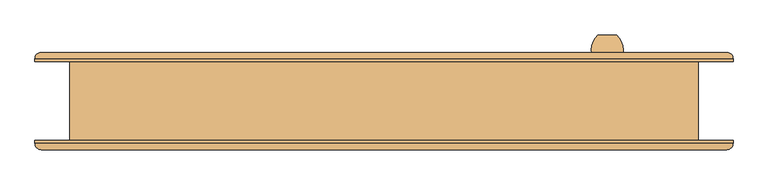
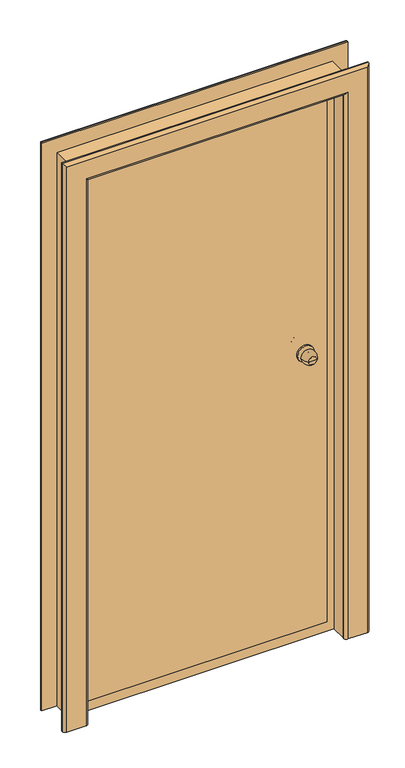
"""IFC4 building model written with IfcOpenShell, lengths in millimetres: door geometry, Наружная дверь 1-Навесная - Один проем наружу с порогом - 31173-2003 : ДСН КЛН  М1 УЗ 2100-1000 ГОСТ 31173-2003 2."""

from ifc_helpers import new_model, si_unit, point, frame, origin, place, context, project, spatial, polyline, circle_curve, ellipse_curve, trimmed, outline, extrude, faceted_brep, source, transform, mapped, element, save
from ifc_brep_helpers import plane_surface, cylinder_surface, revolved_surface, advanced_brep


def door_9195733c(model_context):
    return source(origin(), model_context, "Body", "SolidModel", [
        advanced_brep(
        [(340.0, 105.5, 1100.0), (370.0, 105.5, 1100.0), (355.0, 105.5, 1100.0), (330.0, 75.5, 1100.0), (380.0, 75.5, 1100.0), (337.0, 75.5, 1100.0), (373.0, 75.5, 1100.0), (345.0, 67.5, 1100.0), (365.0, 67.5, 1100.0), (345.0, 61.5, 1100.0), (365.0, 61.5, 1100.0), (385.0, 61.5, 1100.0), (325.0, 61.5, 1100.0), (385.0, 55.5, 1100.0), (325.0, 55.5, 1100.0)],
        [
            (0, 1, circle_curve(frame((355.0, 105.5, 1100.0), z_axis=(0.0, 1.0, 0.0), x_axis=(1.0, 0.0, 0.0)), 15.0)),
            (1, 2),
            (2, 0),
            (1, 0, circle_curve(frame((355.0, 105.5, 1100.0), z_axis=(0.0, 1.0, 0.0), x_axis=(1.0, 0.0, 0.0)), 15.0)),
            (0, 3, circle_curve(frame((364.6226265, 80.6257912, 1100.0), z_axis=(0.0, 0.0, 1.0), x_axis=(1.0, 0.0, 0.0)), 35.0)),
            (3, 4, circle_curve(frame((355.0, 75.5, 1100.0), z_axis=(0.0, 1.0, 0.0), x_axis=(1.0, 0.0, 0.0)), 25.0)),
            (4, 1, circle_curve(frame((345.3773735, 80.6257912, 1100.0), z_axis=(0.0, 0.0, 1.0), x_axis=(-1.0, 0.0, 0.0)), 35.0)),
            (4, 3, circle_curve(frame((355.0, 75.5, 1100.0), z_axis=(0.0, 1.0, 0.0), x_axis=(1.0, 0.0, 0.0)), 25.0)),
            (3, 5),
            (5, 6, circle_curve(frame((355.0, 75.5, 1100.0), z_axis=(0.0, 1.0, 0.0), x_axis=(1.0, 0.0, 0.0)), 18.0)),
            (6, 4),
            (6, 5, circle_curve(frame((355.0, 75.5, 1100.0), z_axis=(0.0, 1.0, 0.0), x_axis=(1.0, 0.0, 0.0)), 18.0)),
            (5, 7, circle_curve(frame((337.0, 67.5, 1100.0), z_axis=(0.0, 0.0, -1.0), x_axis=(1.0, 0.0, 0.0)), 8.0)),
            (7, 8, circle_curve(frame((355.0, 67.5, 1100.0), z_axis=(0.0, 1.0, 0.0), x_axis=(1.0, 0.0, 0.0)), 10.0)),
            (8, 6, circle_curve(frame((373.0, 67.5, 1100.0), z_axis=(0.0, 0.0, -1.0), x_axis=(-1.0, 0.0, 0.0)), 8.0)),
            (8, 7, circle_curve(frame((355.0, 67.5, 1100.0), z_axis=(0.0, 1.0, 0.0), x_axis=(1.0, 0.0, 0.0)), 10.0)),
            (7, 9),
            (9, 10, circle_curve(frame((355.0, 61.5, 1100.0), z_axis=(0.0, 1.0, 0.0), x_axis=(1.0, 0.0, 0.0)), 10.0)),
            (10, 8),
            (10, 9, circle_curve(frame((355.0, 61.5, 1100.0), z_axis=(0.0, 1.0, 0.0), x_axis=(1.0, 0.0, 0.0)), 10.0)),
            (11, 12, circle_curve(frame((355.0, 61.5, 1100.0), z_axis=(0.0, 1.0, 0.0), x_axis=(-1.0, 0.0, 0.0)), 30.0)),
            (12, 11, circle_curve(frame((355.0, 61.5, 1100.0), z_axis=(0.0, 1.0, 0.0), x_axis=(-1.0, 0.0, 0.0)), 30.0)),
            (13, 14, circle_curve(frame((355.0, 55.5, 1100.0), z_axis=(0.0, -1.0, 0.0), x_axis=(-1.0, 0.0, 0.0)), 30.0)),
            (14, 13, circle_curve(frame((355.0, 55.5, 1100.0), z_axis=(0.0, -1.0, 0.0), x_axis=(-1.0, 0.0, 0.0)), 30.0)),
            (11, 13),
            (14, 12),
        ],
        [
            plane_surface(frame((355.0, 105.5, 1100.0), z_axis=(0.0, 1.0, 0.0), x_axis=(1.0, 0.0, 0.0))),
            revolved_surface(trimmed(ellipse_curve(frame((345.3773735, 80.6257912, 1100.0), z_axis=(0.0, 0.0, -1.0), x_axis=(-1.0, 0.0, 0.0)), 35.0, 35.0), [point((370.0, 105.5, 1100.0))], [point((380.0, 75.5, 1100.0))], True, "CARTESIAN"), (355.0, 135.5, 1100.0), (0.0, -1.0, 0.0)),
            plane_surface(frame((355.0, 75.5, 1100.0), z_axis=(0.0, -1.0, 0.0), x_axis=(1.0, 0.0, 0.0))),
            revolved_surface(trimmed(ellipse_curve(frame((373.0, 67.5, 1100.0), z_axis=(0.0, 0.0, 1.0), x_axis=(-1.0, 0.0, 0.0)), 8.0, 8.0), [point((373.0, 75.5, 1100.0))], [point((365.0, 67.5, 1100.0))], True, "CARTESIAN"), (355.0, 135.5, 1100.0), (0.0, -1.0, 0.0)),
            cylinder_surface(frame((355.0, 135.5, 1100.0), z_axis=(0.0, -1.0, 0.0), x_axis=(1.0, 0.0, 0.0)), 10.0),
            plane_surface(frame((325.0, 61.5, 1100.0), z_axis=(0.0, 1.0, 0.0), x_axis=(0.0, 0.0, 1.0))),
            plane_surface(frame((325.0, 55.5, 1100.0), z_axis=(0.0, -1.0, 0.0), x_axis=(0.0, 0.0, -1.0))),
            cylinder_surface(frame((355.0, 55.5, 1100.0), z_axis=(0.0, 1.0, 0.0), x_axis=(-1.0, 0.0, 0.0)), 30.0),
        ],
        [
            (0, [[1, 2, 3]]),
            (0, [[-2, 4, -3]]),
            (1, [[-1, 5, 6, 7]]),
            (1, [[-4, -7, 8, -5]]),
            (2, [[-6, 9, 10, 11]]),
            (2, [[-8, -11, 12, -9]]),
            (3, [[-10, 13, 14, 15]]),
            (3, [[-12, -15, 16, -13]]),
            (4, [[-14, 17, 18, 19]]),
            (4, [[-16, -19, 20, -17]]),
            (5, [[21, 22], [-18, -20]]),
            (6, [[23, 24]]),
            (7, [[-21, 25, -24, 26]]),
            (7, [[-22, -26, -23, -25]]),
        ],
    ),
        advanced_brep(
        [(370.0, -64.5, 1100.0), (340.0, -64.5, 1100.0), (355.0, -64.5, 1100.0), (380.0, -34.5, 1100.0), (330.0, -34.5, 1100.0), (373.0, -34.5, 1100.0), (337.0, -34.5, 1100.0), (365.0, -26.5, 1100.0), (345.0, -26.5, 1100.0), (365.0, -20.5, 1100.0), (345.0, -20.5, 1100.0), (325.0, -20.5, 1100.0), (385.0, -20.5, 1100.0), (325.0, -14.5, 1100.0), (385.0, -14.5, 1100.0)],
        [
            (0, 1, circle_curve(frame((355.0, -64.5, 1100.0), z_axis=(0.0, -1.0, 0.0), x_axis=(-1.0, 0.0, 0.0)), 15.0)),
            (1, 2),
            (2, 0),
            (1, 0, circle_curve(frame((355.0, -64.5, 1100.0), z_axis=(0.0, -1.0, 0.0), x_axis=(-1.0, 0.0, 0.0)), 15.0)),
            (0, 3, circle_curve(frame((345.3773735, -39.6257912, 1100.0), z_axis=(0.0, 0.0, 1.0), x_axis=(-1.0, 0.0, 0.0)), 35.0)),
            (3, 4, circle_curve(frame((355.0, -34.5, 1100.0), z_axis=(0.0, -1.0, 0.0), x_axis=(-1.0, 0.0, 0.0)), 25.0)),
            (4, 1, circle_curve(frame((364.6226265, -39.6257912, 1100.0), z_axis=(0.0, 0.0, 1.0), x_axis=(1.0, 0.0, 0.0)), 35.0)),
            (4, 3, circle_curve(frame((355.0, -34.5, 1100.0), z_axis=(0.0, -1.0, 0.0), x_axis=(-1.0, 0.0, 0.0)), 25.0)),
            (3, 5),
            (5, 6, circle_curve(frame((355.0, -34.5, 1100.0), z_axis=(0.0, -1.0, 0.0), x_axis=(-1.0, 0.0, 0.0)), 18.0)),
            (6, 4),
            (6, 5, circle_curve(frame((355.0, -34.5, 1100.0), z_axis=(0.0, -1.0, 0.0), x_axis=(-1.0, 0.0, 0.0)), 18.0)),
            (5, 7, circle_curve(frame((373.0, -26.5, 1100.0), z_axis=(0.0, 0.0, -1.0), x_axis=(-1.0, 0.0, 0.0)), 8.0)),
            (7, 8, circle_curve(frame((355.0, -26.5, 1100.0), z_axis=(0.0, -1.0, 0.0), x_axis=(-1.0, 0.0, 0.0)), 10.0)),
            (8, 6, circle_curve(frame((337.0, -26.5, 1100.0), z_axis=(0.0, 0.0, -1.0), x_axis=(1.0, 0.0, 0.0)), 8.0)),
            (8, 7, circle_curve(frame((355.0, -26.5, 1100.0), z_axis=(0.0, -1.0, 0.0), x_axis=(-1.0, 0.0, 0.0)), 10.0)),
            (7, 9),
            (9, 10, circle_curve(frame((355.0, -20.5, 1100.0), z_axis=(0.0, -1.0, 0.0), x_axis=(-1.0, 0.0, 0.0)), 10.0)),
            (10, 8),
            (10, 9, circle_curve(frame((355.0, -20.5, 1100.0), z_axis=(0.0, -1.0, 0.0), x_axis=(-1.0, 0.0, 0.0)), 10.0)),
            (11, 12, circle_curve(frame((355.0, -20.5, 1100.0), z_axis=(0.0, -1.0, 0.0), x_axis=(1.0, 0.0, 0.0)), 30.0)),
            (12, 11, circle_curve(frame((355.0, -20.5, 1100.0), z_axis=(0.0, -1.0, 0.0), x_axis=(1.0, 0.0, 0.0)), 30.0)),
            (13, 14, circle_curve(frame((355.0, -14.5, 1100.0), z_axis=(0.0, 1.0, 0.0), x_axis=(1.0, 0.0, 0.0)), 30.0)),
            (14, 13, circle_curve(frame((355.0, -14.5, 1100.0), z_axis=(0.0, 1.0, 0.0), x_axis=(1.0, 0.0, 0.0)), 30.0)),
            (11, 13),
            (14, 12),
        ],
        [
            plane_surface(frame((355.0, -64.5, 1100.0), z_axis=(0.0, -1.0, 0.0), x_axis=(-1.0, 0.0, 0.0))),
            revolved_surface(trimmed(ellipse_curve(frame((364.6226265, -39.6257912, 1100.0), z_axis=(0.0, 0.0, -1.0), x_axis=(1.0, 0.0, 0.0)), 35.0, 35.0), [point((340.0, -64.5, 1100.0))], [point((330.0, -34.5, 1100.0))], True, "CARTESIAN"), (355.0, -94.5, 1100.0), (0.0, 1.0, 0.0)),
            plane_surface(frame((355.0, -34.5, 1100.0), z_axis=(0.0, 1.0, 0.0), x_axis=(-1.0, 0.0, 0.0))),
            revolved_surface(trimmed(ellipse_curve(frame((337.0, -26.5, 1100.0), z_axis=(0.0, 0.0, 1.0), x_axis=(1.0, 0.0, 0.0)), 8.0, 8.0), [point((337.0, -34.5, 1100.0))], [point((345.0, -26.5, 1100.0))], True, "CARTESIAN"), (355.0, -94.5, 1100.0), (0.0, 1.0, 0.0)),
            cylinder_surface(frame((355.0, -94.5, 1100.0), z_axis=(0.0, 1.0, 0.0), x_axis=(-1.0, 0.0, 0.0)), 10.0),
            plane_surface(frame((385.0, -20.5, 1100.0), z_axis=(0.0, -1.0, 0.0), x_axis=(0.0, 0.0, 1.0))),
            plane_surface(frame((385.0, -14.5, 1100.0), z_axis=(0.0, 1.0, 0.0), x_axis=(0.0, 0.0, -1.0))),
            cylinder_surface(frame((355.0, -14.5, 1100.0), z_axis=(0.0, -1.0, 0.0), x_axis=(1.0, 0.0, 0.0)), 30.0),
        ],
        [
            (0, [[1, 2, 3]]),
            (0, [[-2, 4, -3]]),
            (1, [[-1, 5, 6, 7]]),
            (1, [[-4, -7, 8, -5]]),
            (2, [[-6, 9, 10, 11]]),
            (2, [[-8, -11, 12, -9]]),
            (3, [[-10, 13, 14, 15]]),
            (3, [[-12, -15, 16, -13]]),
            (4, [[-14, 17, 18, 19]]),
            (4, [[-16, -19, 20, -17]]),
            (5, [[21, 22], [-18, -20]]),
            (6, [[23, 24]]),
            (7, [[-21, 25, -24, 26]]),
            (7, [[-22, -26, -23, -25]]),
        ],
    ),
        faceted_brep([(435.0, -14.5, 42.0), (-435.0, -14.5, 42.0), (-435.0, -9.5, 42.0), (435.0, -9.5, 42.0), (435.0, -14.5, 2055.0), (435.0, -9.5, 2055.0), (-435.0, -9.5, 2055.0), (415.0, -9.5, 2035.0), (-415.0, -9.5, 2035.0), (-415.0, -9.5, 62.0), (415.0, -9.5, 62.0), (-435.0, -14.5, 2055.0), (415.0, 55.5, 62.0), (415.0, 55.5, 2035.0), (-415.0, 55.5, 62.0), (-415.0, 55.5, 2035.0)], [[[0, 1, 2, 3]], [[4, 0, 3, 5]], [[5, 3, 2, 6], [7, 8, 9, 10]], [[2, 1, 11, 6]], [[11, 1, 0, 4]], [[7, 10, 12, 13]], [[9, 14, 12, 10]], [[15, 14, 9, 8]], [[13, 12, 14, 15]], [[4, 5, 6, 11]], [[7, 13, 15, 8]]]),
        extrude(outline(polyline([(0.0, 480.0), (2100.0, 480.0), (2100.0, -480.0), (0.0, -480.0), (0.0, -465.0), (2085.0, -465.0), (2085.0, 465.0), (0.0, 465.0), (0.0, 480.0)])), frame((0.0, -62.5, 0.0), z_axis=(0.0, 1.0, 0.0), x_axis=(0.0, 0.0, 1.0)), (0.0, 0.0, 1.0), 55.0),
        faceted_brep([(480.0, -7.5, 0.0), (-480.0, -7.5, 0.0), (-480.0, 62.5, 0.0), (480.0, 62.5, 0.0), (-480.0, -7.5, 2100.0), (-480.0, 62.5, 2100.0), (480.0, 62.5, 2100.0), (-400.0, 62.5, 2020.0), (-400.0, 62.5, 80.0), (400.0, 62.5, 80.0), (400.0, 62.5, 2020.0), (480.0, -7.5, 2100.0), (-420.0, -7.5, 60.0), (-420.0, -7.5, 2040.0), (420.0, -7.5, 2040.0), (420.0, -7.5, 60.0), (420.0, 57.5, 60.0), (-420.0, 57.5, 60.0), (-420.0, 57.5, 2040.0), (420.0, 57.5, 2040.0), (-400.0, 57.5, 80.0), (-400.0, 57.5, 2020.0), (400.0, 57.5, 2020.0), (400.0, 57.5, 80.0)], [[[0, 1, 2, 3]], [[1, 4, 5, 2]], [[2, 5, 6, 3], [7, 8, 9, 10]], [[4, 1, 0, 11], [12, 13, 14, 15]], [[16, 17, 12, 15]], [[17, 18, 13, 12]], [[18, 17, 16, 19], [20, 21, 22, 23]], [[9, 8, 20, 23]], [[8, 7, 21, 20]], [[11, 0, 3, 6]], [[19, 16, 15, 14]], [[10, 9, 23, 22]], [[4, 11, 6, 5]], [[18, 19, 14, 13]], [[7, 10, 22, 21]]]),
        advanced_brep(
        [(-555.0, 62.5, 0.0), (-555.0, 67.5, 0.0), (-545.0, 77.5, 0.0), (-475.0, 77.5, 0.0), (-465.0, 67.5, 0.0), (-465.0, 62.5, 0.0), (-465.0, 62.5, 2085.0), (465.0, 62.5, 2085.0), (465.0, 62.5, 0.0), (555.0, 62.5, 0.0), (555.0, 62.5, 2175.0), (-555.0, 62.5, 2175.0), (-465.0, 67.5, 2085.0), (-475.0, 77.5, 2095.0), (-545.0, 77.5, 2165.0), (545.0, 77.5, 2165.0), (545.0, 77.5, 0.0), (475.0, 77.5, 0.0), (475.0, 77.5, 2095.0), (-555.0, 67.5, 2175.0), (555.0, 67.5, 0.0), (555.0, 67.5, 2175.0), (465.0, 67.5, 0.0), (465.0, 67.5, 2085.0)],
        [
            (0, 1),
            (1, 2, circle_curve(frame((-545.0, 67.5, 0.0), z_axis=(0.0, 0.0, -1.0), x_axis=(-1.0, 0.0, 0.0)), 10.0)),
            (2, 3),
            (3, 4, circle_curve(frame((-475.0, 67.5, 0.0), z_axis=(0.0, 0.0, -1.0), x_axis=(-1.0, 0.0, 0.0)), 10.0)),
            (4, 5),
            (5, 0),
            (5, 6),
            (6, 7),
            (7, 8),
            (8, 9),
            (9, 10),
            (10, 11),
            (11, 0),
            (4, 12),
            (12, 6),
            (3, 13),
            (13, 12, ellipse_curve(frame((-475.0, 67.5, 2095.0), z_axis=(-0.7071067811865475, 0.0, -0.7071067811865475), x_axis=(0.7071067811865474, 0.0, -0.7071067811865476)), 14.1421356, 10.0)),
            (2, 14),
            (14, 15),
            (15, 16),
            (16, 17),
            (17, 18),
            (18, 13),
            (1, 19),
            (19, 14, ellipse_curve(frame((-545.0, 67.5, 2165.0), z_axis=(-0.7071067811865475, 0.0, -0.7071067811865475), x_axis=(0.7071067811865474, 0.0, -0.7071067811865476)), 14.1421356, 10.0)),
            (11, 19),
            (9, 20),
            (20, 21),
            (21, 10),
            (8, 22),
            (22, 17, circle_curve(frame((475.0, 67.5, 0.0), z_axis=(0.0, 0.0, -1.0), x_axis=(1.0, 0.0, 0.0)), 10.0)),
            (16, 20, circle_curve(frame((545.0, 67.5, 0.0), z_axis=(0.0, 0.0, -1.0), x_axis=(1.0, 0.0, 0.0)), 10.0)),
            (23, 22),
            (7, 23),
            (23, 18, ellipse_curve(frame((475.0, 67.5, 2095.0), z_axis=(0.7071067811865475, 0.0, -0.7071067811865475), x_axis=(0.7071067811865474, 0.0, 0.7071067811865476)), 14.1421356, 10.0)),
            (15, 21, ellipse_curve(frame((545.0, 67.5, 2165.0), z_axis=(0.7071067811865475, 0.0, -0.7071067811865475), x_axis=(0.7071067811865474, 0.0, 0.7071067811865476)), 14.1421356, 10.0)),
            (12, 23),
            (19, 21),
        ],
        [
            plane_surface(frame((-500.0, 62.5, 0.0), z_axis=(0.0, 0.0, -1.0), x_axis=(0.0, 1.0, 0.0))),
            plane_surface(frame((-555.0, 62.5, 0.0), z_axis=(0.0, -1.0, 0.0), x_axis=(0.0, 0.0, 1.0))),
            plane_surface(frame((-465.0, 62.5, 0.0), z_axis=(1.0, 0.0, 0.0), x_axis=(0.0, 0.0, 1.0))),
            cylinder_surface(frame((-475.0, 67.5, 0.0), z_axis=(0.0, 0.0, -1.0), x_axis=(-1.0, 0.0, 0.0)), 10.0),
            plane_surface(frame((-475.0, 77.5, 0.0), z_axis=(0.0, 1.0, 0.0), x_axis=(0.0, 0.0, 1.0))),
            cylinder_surface(frame((-545.0, 67.5, 0.0), z_axis=(0.0, 0.0, -1.0), x_axis=(-1.0, 0.0, 0.0)), 10.0),
            plane_surface(frame((-555.0, 67.5, 0.0), z_axis=(-1.0, 0.0, 0.0), x_axis=(0.0, 0.0, 1.0))),
            plane_surface(frame((555.0, 67.5, 2175.0), z_axis=(1.0, 0.0, 0.0), x_axis=(0.0, 0.0, -1.0))),
            plane_surface(frame((500.0, 62.5, 0.0), z_axis=(0.0, 0.0, -1.0), x_axis=(0.0, 1.0, 0.0))),
            plane_surface(frame((465.0, 62.5, 2085.0), z_axis=(-1.0, 0.0, 0.0), x_axis=(0.0, 0.0, -1.0))),
            cylinder_surface(frame((475.0, 67.5, 2120.0), z_axis=(0.0, 0.0, 1.0), x_axis=(1.0, 0.0, 0.0)), 10.0),
            cylinder_surface(frame((545.0, 67.5, 2120.0), z_axis=(0.0, 0.0, 1.0), x_axis=(1.0, 0.0, 0.0)), 10.0),
            plane_surface(frame((-465.0, 62.5, 2085.0), z_axis=(0.0, 0.0, -1.0), x_axis=(1.0, 0.0, 0.0))),
            cylinder_surface(frame((-500.0, 67.5, 2095.0), z_axis=(-1.0, 0.0, 0.0), x_axis=(0.0, 0.0, 1.0)), 10.0),
            cylinder_surface(frame((-500.0, 67.5, 2165.0), z_axis=(-1.0, 0.0, 0.0), x_axis=(0.0, 0.0, 1.0)), 10.0),
            plane_surface(frame((-555.0, 67.5, 2175.0), z_axis=(0.0, 0.0, 1.0), x_axis=(1.0, 0.0, 0.0))),
        ],
        [
            (0, [[1, 2, 3, 4, 5, 6]]),
            (1, [[7, 8, 9, 10, 11, 12, 13, -6]]),
            (2, [[14, 15, -7, -5]]),
            (3, [[16, 17, -14, -4]]),
            (4, [[18, 19, 20, 21, 22, 23, -16, -3]]),
            (5, [[24, 25, -18, -2]]),
            (6, [[-13, 26, -24, -1]]),
            (7, [[-11, 27, 28, 29]]),
            (8, [[-10, 30, 31, -21, 32, -27]]),
            (9, [[33, -30, -9, 34]]),
            (10, [[-22, -31, -33, 35]]),
            (11, [[-28, -32, -20, 36]]),
            (12, [[37, -34, -8, -15]]),
            (13, [[-23, -35, -37, -17]]),
            (14, [[38, -36, -19, -25]]),
            (15, [[-12, -29, -38, -26]]),
        ],
    ),
        advanced_brep(
        [(555.0, -62.5, 0.0), (555.0, -67.5, 0.0), (545.0, -77.5, 0.0), (475.0, -77.5, 0.0), (465.0, -67.5, 0.0), (465.0, -62.5, 0.0), (465.0, -62.5, 2085.0), (-465.0, -62.5, 2085.0), (-465.0, -62.5, 0.0), (-555.0, -62.5, 0.0), (-555.0, -62.5, 2175.0), (555.0, -62.5, 2175.0), (465.0, -67.5, 2085.0), (475.0, -77.5, 2095.0), (545.0, -77.5, 2165.0), (-545.0, -77.5, 2165.0), (-545.0, -77.5, 0.0), (-475.0, -77.5, 0.0), (-475.0, -77.5, 2095.0), (555.0, -67.5, 2175.0), (-555.0, -67.5, 0.0), (-555.0, -67.5, 2175.0), (-465.0, -67.5, 0.0), (-465.0, -67.5, 2085.0)],
        [
            (0, 1),
            (1, 2, circle_curve(frame((545.0, -67.5, 0.0), z_axis=(0.0, 0.0, -1.0), x_axis=(1.0, 0.0, 0.0)), 10.0)),
            (2, 3),
            (3, 4, circle_curve(frame((475.0, -67.5, 0.0), z_axis=(0.0, 0.0, -1.0), x_axis=(1.0, 0.0, 0.0)), 10.0)),
            (4, 5),
            (5, 0),
            (5, 6),
            (6, 7),
            (7, 8),
            (8, 9),
            (9, 10),
            (10, 11),
            (11, 0),
            (4, 12),
            (12, 6),
            (3, 13),
            (13, 12, ellipse_curve(frame((475.0, -67.5, 2095.0), z_axis=(0.7071067811865475, 0.0, -0.7071067811865475), x_axis=(-0.7071067811865474, 0.0, -0.7071067811865476)), 14.1421356, 10.0)),
            (2, 14),
            (14, 15),
            (15, 16),
            (16, 17),
            (17, 18),
            (18, 13),
            (1, 19),
            (19, 14, ellipse_curve(frame((545.0, -67.5, 2165.0), z_axis=(0.7071067811865475, 0.0, -0.7071067811865475), x_axis=(-0.7071067811865474, 0.0, -0.7071067811865476)), 14.1421356, 10.0)),
            (11, 19),
            (9, 20),
            (20, 21),
            (21, 10),
            (8, 22),
            (22, 17, circle_curve(frame((-475.0, -67.5, 0.0), z_axis=(0.0, 0.0, -1.0), x_axis=(-1.0, 0.0, 0.0)), 10.0)),
            (16, 20, circle_curve(frame((-545.0, -67.5, 0.0), z_axis=(0.0, 0.0, -1.0), x_axis=(-1.0, 0.0, 0.0)), 10.0)),
            (23, 22),
            (7, 23),
            (23, 18, ellipse_curve(frame((-475.0, -67.5, 2095.0), z_axis=(-0.7071067811865475, 0.0, -0.7071067811865475), x_axis=(-0.7071067811865474, 0.0, 0.7071067811865476)), 14.1421356, 10.0)),
            (15, 21, ellipse_curve(frame((-545.0, -67.5, 2165.0), z_axis=(-0.7071067811865475, 0.0, -0.7071067811865475), x_axis=(-0.7071067811865474, 0.0, 0.7071067811865476)), 14.1421356, 10.0)),
            (12, 23),
            (19, 21),
        ],
        [
            plane_surface(frame((500.0, -62.5, 0.0), z_axis=(0.0, 0.0, -1.0), x_axis=(0.0, 1.0, 0.0))),
            plane_surface(frame((555.0, -62.5, 0.0), z_axis=(0.0, 1.0, 0.0), x_axis=(0.0, 0.0, 1.0))),
            plane_surface(frame((465.0, -62.5, 0.0), z_axis=(-1.0, 0.0, 0.0), x_axis=(0.0, 0.0, 1.0))),
            cylinder_surface(frame((475.0, -67.5, 0.0), z_axis=(0.0, 0.0, -1.0), x_axis=(1.0, 0.0, 0.0)), 10.0),
            plane_surface(frame((475.0, -77.5, 0.0), z_axis=(0.0, -1.0, 0.0), x_axis=(0.0, 0.0, 1.0))),
            cylinder_surface(frame((545.0, -67.5, 0.0), z_axis=(0.0, 0.0, -1.0), x_axis=(1.0, 0.0, 0.0)), 10.0),
            plane_surface(frame((555.0, -67.5, 0.0), z_axis=(1.0, 0.0, 0.0), x_axis=(0.0, 0.0, 1.0))),
            plane_surface(frame((-555.0, -67.5, 2175.0), z_axis=(-1.0, 0.0, 0.0), x_axis=(0.0, 0.0, -1.0))),
            plane_surface(frame((-500.0, -62.5, 0.0), z_axis=(0.0, 0.0, -1.0), x_axis=(0.0, 1.0, 0.0))),
            plane_surface(frame((-465.0, -62.5, 2085.0), z_axis=(1.0, 0.0, 0.0), x_axis=(0.0, 0.0, -1.0))),
            cylinder_surface(frame((-475.0, -67.5, 2120.0), z_axis=(0.0, 0.0, 1.0), x_axis=(-1.0, 0.0, 0.0)), 10.0),
            cylinder_surface(frame((-545.0, -67.5, 2120.0), z_axis=(0.0, 0.0, 1.0), x_axis=(-1.0, 0.0, 0.0)), 10.0),
            plane_surface(frame((465.0, -62.5, 2085.0), z_axis=(0.0, 0.0, -1.0), x_axis=(-1.0, 0.0, 0.0))),
            cylinder_surface(frame((500.0, -67.5, 2095.0), z_axis=(1.0, 0.0, 0.0), x_axis=(0.0, 0.0, 1.0)), 10.0),
            cylinder_surface(frame((500.0, -67.5, 2165.0), z_axis=(1.0, 0.0, 0.0), x_axis=(0.0, 0.0, 1.0)), 10.0),
            plane_surface(frame((555.0, -67.5, 2175.0), z_axis=(0.0, 0.0, 1.0), x_axis=(-1.0, 0.0, 0.0))),
        ],
        [
            (0, [[1, 2, 3, 4, 5, 6]]),
            (1, [[7, 8, 9, 10, 11, 12, 13, -6]]),
            (2, [[14, 15, -7, -5]]),
            (3, [[16, 17, -14, -4]]),
            (4, [[18, 19, 20, 21, 22, 23, -16, -3]]),
            (5, [[24, 25, -18, -2]]),
            (6, [[-13, 26, -24, -1]]),
            (7, [[-11, 27, 28, 29]]),
            (8, [[-10, 30, 31, -21, 32, -27]]),
            (9, [[33, -30, -9, 34]]),
            (10, [[-22, -31, -33, 35]]),
            (11, [[-28, -32, -20, 36]]),
            (12, [[37, -34, -8, -15]]),
            (13, [[-23, -35, -37, -17]]),
            (14, [[38, -36, -19, -25]]),
            (15, [[-12, -29, -38, -26]]),
        ],
    ),
        extrude(outline(polyline([(0.0, 500.0), (2120.0, 500.0), (2120.0, -500.0), (0.0, -500.0), (0.0, -480.0), (2100.0, -480.0), (2100.0, 480.0), (0.0, 480.0), (0.0, 500.0)])), frame((0.0, -62.5, 0.0), z_axis=(0.0, 1.0, 0.0), x_axis=(0.0, 0.0, 1.0)), (0.0, 0.0, 1.0), 125.0),
    ])


if __name__ == "__main__":
    model = new_model("IFC4")
    model_context = context("Model", 3, world=origin())
    ifc_project = project(units=[si_unit("LENGTHUNIT", "METRE", prefix="MILLI")], contexts=[model_context])
    site = spatial("IfcSite", under=ifc_project)
    building = spatial("IfcBuilding", under=site)
    placement = place(None, origin())
    door_shape = door_9195733c(model_context)
    element("IfcDoor", 1, ObjectType="Наружная дверь 1-Навесная - Один проем наружу с порогом - 31173-2003 : ДСН КЛН  М1 УЗ 2100-1000 ГОСТ 31173-2003 2", at=placement, inside=building, context=model_context, shape_type="MappedRepresentation", body=[
        mapped(door_shape, transform((0.0, 0.0, 0.0), x_axis=(1.0, 0.0, 0.0), y_axis=(0.0, 1.0, 0.0), z_axis=(0.0, 0.0, 1.0))),
    ])
    save(model, "model.ifc")

# Revit data of these elements
# Type "Наружная дверь 1-Навесная - Один проем наружу с порогом - 31173-2003 : ДСН КЛН  М1 УЗ 2100-1000 ГОСТ 31173-2003 2"
#   Type Mark = "149"
#   Description = "ДСН КЛН  М1 УЗ 2100-900 ГОСТ 31173-2003"
#   Проекционное соединение по ширине = 90 mm
#   Rough Width = 1000 mm
#   Rough Height = 2120 mm
#   Угол проема [instance default] = 30°
#   Толщина_Тепл_Изоляции = 20 mm
#   Heat Transfer Coefficient (U) = 3.7021 W/(m²·K)
#   Height = 2100 mm
#   Width = 960 mm
#   Ширина каркаса = 60 mm
#   Толщина каркаса = 70 mm
#   Вставка двери [instance default] = 0 mm
#   Правая сторона = no
#   Левая сторона = yes
#   Function = 1
#   Обрезка = Сталь
#   Панель = Сталь
#   Тепловая изоляция = Тепловая изоляция
#   Кадр = Сталь
#   Дверная ручка = Металл
#   Visual Light Transmittance = 0
#   Solar Heat Gain Coefficient = 0
#   Construction Type Id = ""
#   Wall Closure = (empty or 0)
#   Analytic Construction = (empty or 0)
# Element 1 (IfcDoor, "Наружная дверь 1-Навесная - Один проем наружу с порогом - 31173-2003 : ДСН КЛН  М1 УЗ 2100-1000 ГОСТ 31173-2003 2")
#   Materials on its faces: "Сталь", "Металл", "Тепловая изоляция"
# Materials
#   "Сталь": class "Металл", colour RGB 247 247 247, transparency 0
#   "Тепловая изоляция": class "Пластмасса", colour RGB 185 154 119, transparency 0, Cost = 0
#   "Металл": class "Металл", colour RGB 249 249 249, transparency 0
